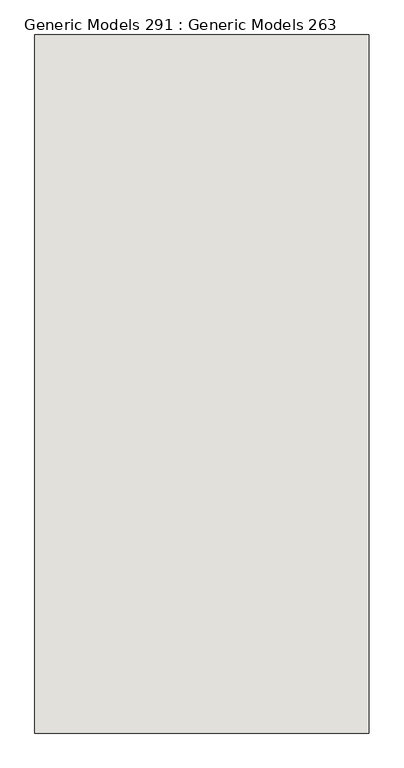
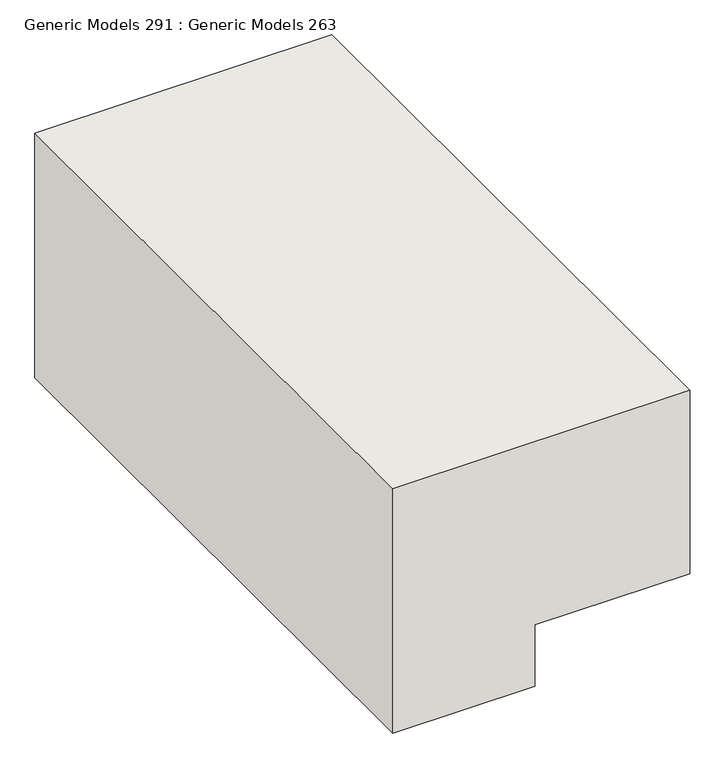
"""IFC4 building model written with IfcOpenShell, lengths in millimetres: wall geometry, Generic Models 291 : Generic Models 263."""

import ifcopenshell
import ifcopenshell.guid

model = None  # the IFC model being written
_history = None  # IfcOwnerHistory: only IFC2X3 demands one
_inside = {}  # id of a spatial element -> (the spatial element, [elements in it])
_under = {}  # id of a project, library or spatial element -> (it, [spatial elements below it])
_declared = {}  # id of a project -> (the project, [libraries it declares])
_typed = {}  # id of a type object -> (the type object, [elements of that type])
_made_of = {}  # id of a material, layer set ... -> (it, [elements and type objects made of it])


def new_model(schema):
    """Start an empty IFC model of exactly this schema.

    Asked for "IFC4X3", IfcOpenShell would pick the latest addendum, in which some entities
    have other attributes; the version numbers below select the first issue.
    IFC2X3 requires an IfcOwnerHistory on every rooted entity: one is made here for all.
    """
    global model, _history
    if schema == "IFC4X3":
        model = ifcopenshell.file(schema_version=(4, 3, 0, 0))
    else:
        model = ifcopenshell.file(schema=schema)
    _inside.clear()
    _under.clear()
    _declared.clear()
    _typed.clear()
    _made_of.clear()
    _history = None
    if model.schema == "IFC2X3":
        org = make("IfcOrganization", Name="unknown")
        user = make(
            "IfcPersonAndOrganization",
            ThePerson=make("IfcPerson", FamilyName="unknown"),
            TheOrganization=org,
        )
        app = make(
            "IfcApplication",
            ApplicationDeveloper=org,
            Version="unknown",
            ApplicationFullName="unknown",
            ApplicationIdentifier="unknown",
        )
        _history = make(
            "IfcOwnerHistory",
            OwningUser=user,
            OwningApplication=app,
            ChangeAction="ADDED",
            CreationDate=0,
        )
    return model


def make(cls, **values):
    """One entity of the class cls with the attributes given. An attribute that is None is left unset."""
    return model.create_entity(
        cls, **{name: value for name, value in values.items() if value is not None}
    )


def rooted(cls, **values):
    """An entity with a GlobalId (a new one), such as an element, a storey or a relation."""
    return make(cls, GlobalId=ifcopenshell.guid.new(), OwnerHistory=_history, **values)


def si_unit(unit_type, name, prefix=None):
    """IfcSIUnit, for example si_unit("LENGTHUNIT", "METRE", prefix="MILLI")."""
    return make("IfcSIUnit", UnitType=unit_type, Prefix=prefix, Name=name)


def assignment(units):
    """IfcUnitAssignment: the units of a project."""
    return None if units is None else make("IfcUnitAssignment", Units=units)


def point(xyz):
    """IfcCartesianPoint."""
    return None if xyz is None else make("IfcCartesianPoint", Coordinates=xyz)


def direction(xyz):
    """IfcDirection."""
    return None if xyz is None else make("IfcDirection", DirectionRatios=xyz)


def frame(location, z_axis=None, x_axis=None):
    """IfcAxis2Placement3D, a coordinate frame: its origin and axes. An axis left out is left unset."""
    return make(
        "IfcAxis2Placement3D",
        Location=point(location),
        Axis=direction(z_axis),
        RefDirection=direction(x_axis),
    )


def origin():
    """The frame at (0, 0, 0) with its axes left unset."""
    return frame((0.0, 0.0, 0.0))


def place(relative_to, where):
    """IfcLocalPlacement: puts the frame where relative to a parent placement (None: the world)."""
    return make(
        "IfcLocalPlacement", PlacementRelTo=relative_to, RelativePlacement=where
    )


def context(
    kind, dimensions, precision=None, world=None, true_north=None, identifier=None
):
    """IfcGeometricRepresentationContext, for example the 3D "Model" context."""
    return make(
        "IfcGeometricRepresentationContext",
        ContextIdentifier=identifier,
        ContextType=kind,
        CoordinateSpaceDimension=dimensions,
        Precision=precision,
        WorldCoordinateSystem=world,
        TrueNorth=true_north,
    )


def project(units=None, contexts=None):
    """IfcProject with its units and contexts."""
    return rooted(
        "IfcProject",
        Name="project",
        RepresentationContexts=contexts,
        UnitsInContext=assignment(units),
    )


def spatial(cls, under=None, at=None, **own):
    """A site, building, storey or space (cls), placed at a placement, below another one or the project."""
    s = rooted(cls, ObjectPlacement=at, **own)
    if under is not None:
        _under.setdefault(under.id(), (under, []))[1].append(s)
    return s


def polyline(points):
    """IfcPolyline through the points."""
    return make("IfcPolyline", Points=[point(p) for p in points])


def outline(outer, holes=None, kind="AREA"):
    """IfcArbitraryClosedProfileDef: a profile drawn as a closed curve; with holes, ...WithVoids."""
    if holes is None:
        return make("IfcArbitraryClosedProfileDef", ProfileType=kind, OuterCurve=outer)
    return make(
        "IfcArbitraryProfileDefWithVoids",
        ProfileType=kind,
        OuterCurve=outer,
        InnerCurves=holes,
    )


def extrude(swept, where, along, depth):
    """IfcExtrudedAreaSolid: the profile swept, set in the frame where, extruded along a direction by depth."""
    return make(
        "IfcExtrudedAreaSolid",
        SweptArea=swept,
        Position=where,
        ExtrudedDirection=direction(along),
        Depth=depth,
    )


def shape(context_of_items, identifier, shape_type, items):
    """IfcShapeRepresentation: the items that make up one representation, for example the "Body"."""
    return make(
        "IfcShapeRepresentation",
        ContextOfItems=context_of_items,
        RepresentationIdentifier=identifier,
        RepresentationType=shape_type,
        Items=items,
    )


def source(mapping_origin, context_of_items, identifier, shape_type, items):
    """IfcRepresentationMap: a shape defined once, which mapped items show again and again."""
    return make(
        "IfcRepresentationMap",
        MappingOrigin=mapping_origin,
        MappedRepresentation=shape(context_of_items, identifier, shape_type, items),
    )


def transform(
    local_origin,
    x_axis=None,
    y_axis=None,
    z_axis=None,
    scale=None,
    scale2=None,
    scale3=None,
    uniform=True,
):
    """IfcCartesianTransformationOperator3D, or its non-uniform kind. x_axis, y_axis, z_axis: its Axis1, 2, 3."""
    if uniform:
        return make(
            "IfcCartesianTransformationOperator3D",
            Axis1=direction(x_axis),
            Axis2=direction(y_axis),
            LocalOrigin=point(local_origin),
            Scale=scale,
            Axis3=direction(z_axis),
        )
    return make(
        "IfcCartesianTransformationOperator3DnonUniform",
        Axis1=direction(x_axis),
        Axis2=direction(y_axis),
        LocalOrigin=point(local_origin),
        Scale=scale,
        Axis3=direction(z_axis),
        Scale2=scale2,
        Scale3=scale3,
    )


def mapped(mapping_source, mapping_target):
    """IfcMappedItem: shows the shape of a source again, moved by a transform."""
    return make(
        "IfcMappedItem", MappingSource=mapping_source, MappingTarget=mapping_target
    )


def made_of(thing, what):
    """Note that an element or type object is made of a material, layer set ...; save() writes the relation."""
    if what is not None:
        _made_of.setdefault(what.id(), (what, []))[1].append(thing)
    return thing


def element(
    cls,
    number,
    at=None,
    inside=None,
    cuts=None,
    type_object=None,
    material=None,
    context=None,
    identifier="Body",
    shape_type=None,
    held_by="IfcProductDefinitionShape",
    body=None,
    shapes=None,
    **own,
):
    """One element of the class cls, such as IfcWall. Its Tag is "e" and its number.

    at: its placement. inside: the storey or other place that contains it. cuts: it is an
    opening in that element (IfcRelVoidsElement). A single representation is given by context,
    identifier, shape_type and body (its items); several are given by shapes. held_by: the class
    of the entity that holds the representations. save() writes the other relations.
    """
    e = rooted(cls, Tag="e%d" % number, ObjectPlacement=at, **own)
    if body is not None:
        shapes = [shape(context, identifier, shape_type, body)]
    if shapes is not None:
        e.Representation = make(held_by, Representations=shapes)
    if inside is not None:
        _inside.setdefault(inside.id(), (inside, []))[1].append(e)
    if cuts is not None:
        rooted(
            "IfcRelVoidsElement", RelatingBuildingElement=cuts, RelatedOpeningElement=e
        )
    if type_object is not None:
        _typed.setdefault(type_object.id(), (type_object, []))[1].append(e)
    return made_of(e, material)


def aggregate(whole, parts):
    """IfcRelAggregates: a whole, such as a stair, and the parts it consists of."""
    return rooted("IfcRelAggregates", RelatingObject=whole, RelatedObjects=parts)


def save(model, path):
    """Write the relations noted so far, then the file.

    IfcRelAggregates (storeys below a building ...), IfcRelContainedInSpatialStructure (elements
    in a storey), IfcRelDefinesByType, IfcRelAssociatesMaterial and IfcRelDeclares: one each for
    every whole, place, type object, material and project.
    """
    for whole, parts in _under.values():
        aggregate(whole, parts)
    for where, things in _inside.values():
        rooted(
            "IfcRelContainedInSpatialStructure",
            RelatedElements=things,
            RelatingStructure=where,
        )
    for kind, things in _typed.values():
        rooted("IfcRelDefinesByType", RelatedObjects=things, RelatingType=kind)
    for what, things in _made_of.values():
        rooted("IfcRelAssociatesMaterial", RelatedObjects=things, RelatingMaterial=what)
    for by, libraries in _declared.values():
        rooted("IfcRelDeclares", RelatingContext=by, RelatedDefinitions=libraries)
    model.write(path)


def generic_models_291_generic_models_263_452afd1b(model_context):
    return source(origin(), model_context, "Body", "SweptSolid", [
        extrude(outline(polyline([(-381.0, 62319.1797726), (0.0, 62319.1797726), (0.0, 61734.9797726), (-508.0, 61734.9797726), (-508.0, 62014.3797726), (-381.0, 62014.3797726), (-381.0, 62319.1797726)])), frame((0.0, -94.4486541, 0.0), z_axis=(0.0, 1.0, 0.0), x_axis=(0.0, 0.0, 1.0)), (0.0, 0.0, 1.0), 1219.2),
    ])


if __name__ == "__main__":
    model = new_model("IFC4")
    model_context = context("Model", 3, world=origin())
    ifc_project = project(units=[si_unit("LENGTHUNIT", "METRE", prefix="MILLI")], contexts=[model_context])
    site = spatial("IfcSite", under=ifc_project)
    building = spatial("IfcBuilding", under=site)
    placement = place(None, origin())
    generic_models_291_generic_models_263_shape = generic_models_291_generic_models_263_452afd1b(model_context)
    element("IfcWall", 1, ObjectType="Generic Models 291 : Generic Models 263", at=placement, inside=building, context=model_context, shape_type="MappedRepresentation", body=[
        mapped(generic_models_291_generic_models_263_shape, transform((0.0, 0.0, 0.0), x_axis=(1.0, 0.0, 0.0), y_axis=(0.0, 1.0, 0.0), z_axis=(0.0, 0.0, 1.0))),
    ])
    save(model, "model.ifc")

# Revit data of these elements
# Element 1 (IfcWall, "Generic Models 291 : Generic Models 263")
#   Materials on its faces: "GRADED BACKFILL"
# Materials
#   "GRADED BACKFILL": class "Miscellaneous", colour RGB 128 97 77, transparency 0, Cost = 0
